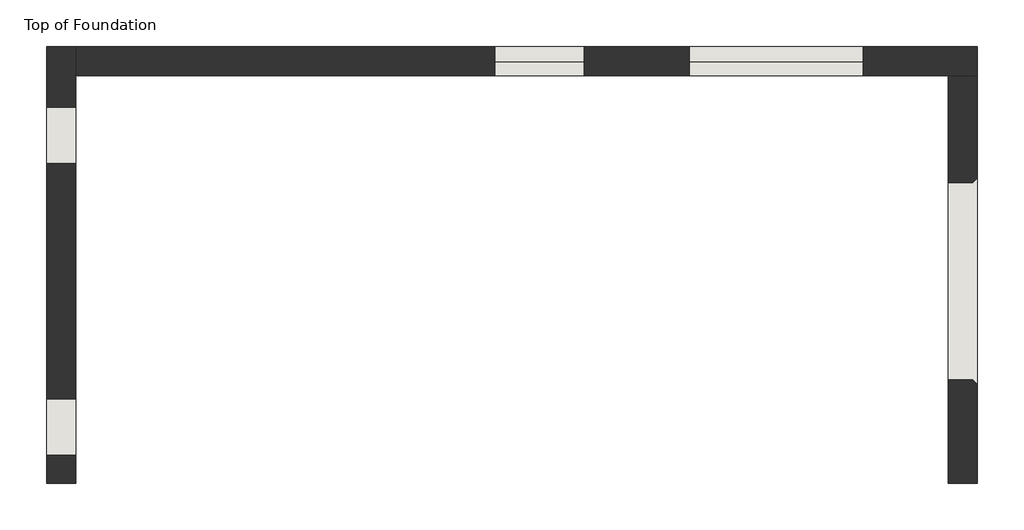
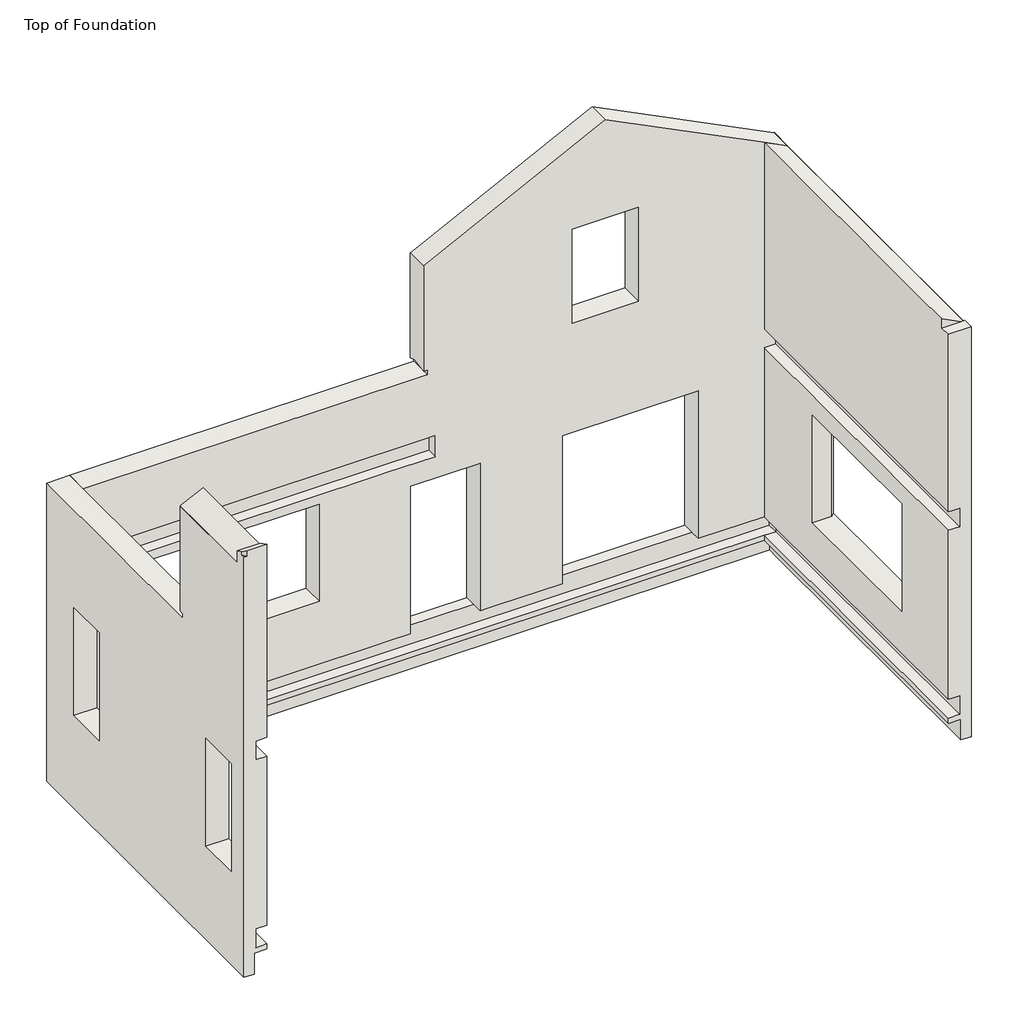
# One storey: 3 walls.
"""IFC4 building model written with IfcOpenShell, lengths in millimetres."""

from ifc_helpers import new_model, si_unit, origin, place, context, project, spatial, faceted_brep, element, save

model = new_model("IFC4")

# Units and contexts
model_context = context("Model", 3, world=origin())
ifc_project = project(units=[si_unit("LENGTHUNIT", "METRE", prefix="MILLI")], contexts=[model_context])

# Site, building, storey
site = spatial("IfcSite", under=ifc_project)
building = spatial("IfcBuilding", under=site)
storey = spatial("IfcBuildingStorey", under=building, Name="Top of Foundation", Elevation=-349.25)

# Walls
placement = place(None, origin())
element("IfcWall", 1, ObjectType="Exterior - Brick on Mtl. Stud", at=placement, inside=storey, context=model_context, shape_type="Brep", body=[
    faceted_brep([(-5671.6803068, 3152.0888758, -349.25), (-5671.6803068, 7558.9888758, -349.25), (-5671.6803068, 7876.4888758, -349.25), (-5671.6803068, 7876.4888758, 3708.4), (-5671.6803068, 7558.9888758, 3708.4), (-5671.6803068, 4676.0888758, 3708.4), (-5671.6803068, 4612.5888758, 3708.4), (-5671.6803068, 4612.5888758, 3774.0166667), (-5671.6803068, 4676.0888758, 3774.0166667), (-5671.6803068, 4676.0888758, 5468.9375), (-5671.6803068, 4358.5888758, 5468.9375), (-5671.6803068, 3304.4888758, 5468.9375), (-5671.6803068, 3304.4888758, 5488.5342644), (-5671.6803068, 3152.0888758, 5564.7342644), (-5671.6803068, 3152.0888758, 2743.2), (-5671.6803068, 4358.5888758, 2743.2), (-5671.6803068, 4514.1638758, 2743.2), (-5671.6803068, 4514.1638758, 2781.3), (-5671.6803068, 4676.0888758, 2781.3), (-5671.6803068, 7558.9888758, 2781.3), (-5671.6803068, 7714.5638758, 2781.3), (-5671.6803068, 7714.5638758, 2470.15), (-5671.6803068, 7558.9888758, 2470.15), (-5671.6803068, 3152.0888758, 2470.15), (-5671.6803068, 3152.0888758, 0.0), (-5671.6803068, 7558.9888758, 0.0), (-5671.6803068, 7714.5638758, 0.0), (-5671.6803068, 7714.5638758, -273.05), (-5671.6803068, 7558.9888758, -273.05), (-5671.6803068, 3152.0888758, -273.05), (-5671.6803068, 3456.8888758, 711.2), (-5671.6803068, 3456.8888758, 2286.0), (-5671.6803068, 4066.4888758, 2286.0), (-5671.6803068, 4066.4888758, 711.2), (-5671.6803068, 6609.6638758, 711.2), (-5671.6803068, 6609.6638758, 2286.0), (-5671.6803068, 7219.2638758, 2286.0), (-5671.6803068, 7219.2638758, 711.2), (-5989.1803068, 3152.0888758, -654.05), (-5989.1803068, 3152.0888758, 5486.4), (-5989.1803068, 3199.7138758, 5486.4), (-5989.1803068, 3199.7138758, 5540.9217644), (-5989.1803068, 3304.4888758, 5488.5342644), (-5989.1803068, 3304.4888758, 5312.3217644), (-5989.1803068, 4676.0888758, 5312.3217644), (-5989.1803068, 4676.0888758, 3779.52), (-5989.1803068, 4612.5888758, 3779.52), (-5989.1803068, 4612.5888758, 3708.4), (-5989.1803068, 7876.4888758, 3708.4), (-5989.1803068, 7876.4888758, -654.05), (-5989.1803068, 3456.8888758, 2286.0), (-5989.1803068, 3456.8888758, 711.2), (-5989.1803068, 4066.4888758, 711.2), (-5989.1803068, 4066.4888758, 2286.0), (-5989.1803068, 6609.6638758, 2286.0), (-5989.1803068, 6609.6638758, 711.2), (-5989.1803068, 7219.2638758, 711.2), (-5989.1803068, 7219.2638758, 2286.0), (-5846.3053068, 3152.0888758, -654.05), (-5846.3053068, 3152.0888758, -349.25), (-5684.3803068, 3152.0888758, -349.25), (-5827.2553068, 3152.0888758, -273.05), (-5827.2553068, 3152.0888758, 0.0), (-5827.2553068, 3152.0888758, 2470.15), (-5827.2553068, 3152.0888758, 2743.2), (-5941.5553068, 3152.0888758, 5564.7342644), (-5941.5553068, 3152.0888758, 5486.4), (-5984.911778, 4676.0888758, 5312.3217644), (-5887.5803068, 4676.0888758, 3810.0), (-5846.3053068, 7876.4888758, -349.25), (-5846.3053068, 7876.4888758, -654.05), (-5937.286778, 3304.4888758, 5336.1342644), (-5984.911778, 3304.4888758, 5312.3217644), (-5846.3053068, 7733.6138758, -349.25), (-5846.3053068, 7733.6138758, -654.05), (-5827.2553068, 7714.5638758, -273.05), (-5827.2553068, 7714.5638758, 0.0), (-5827.2553068, 7714.5638758, 2470.15), (-5827.2553068, 4514.1638758, 2470.15), (-5827.2553068, 4514.1638758, 2743.2), (-5827.2553068, 7714.5638758, 2781.3), (-5827.2553068, 4514.1638758, 2781.3), (-5887.5803068, 4612.5888758, 3810.0)], [[[0, 1, 2, 3, 4, 5, 6, 7, 8, 9, 10, 11, 12, 13, 14, 15, 16, 17, 18, 19, 20, 21, 22, 23, 24, 25, 26, 27, 28, 29], [30, 31, 32, 33], [34, 35, 36, 37]], [[38, 39, 40, 41, 42, 43, 44, 45, 46, 47, 48, 49], [50, 51, 52, 53], [54, 55, 56, 57]], [[39, 38, 58, 59, 60, 0, 29, 61, 62, 24, 23, 63, 64, 14, 13, 65, 66]], [[3, 48, 47, 6, 5, 4]], [[67, 9, 8, 68, 45, 44]], [[3, 2, 69, 70, 49, 48]], [[43, 42, 12, 11, 71, 72]], [[40, 39, 66]], [[40, 66, 65, 41]], [[11, 10, 9, 67, 72, 71]], [[44, 43, 72, 67]], [[13, 12, 42, 41, 65]], [[2, 1, 0, 60, 59, 73, 69]], [[69, 73, 59, 58, 74, 70]], [[58, 38, 49, 70, 74]], [[51, 50, 31, 30]], [[52, 51, 30, 33]], [[53, 52, 33, 32]], [[50, 53, 32, 31]], [[55, 54, 35, 34]], [[56, 55, 34, 37]], [[57, 56, 37, 36]], [[54, 57, 36, 35]], [[75, 61, 29, 28, 27]], [[76, 26, 25, 24, 62]], [[76, 75, 27, 26]], [[75, 76, 62, 61]], [[63, 23, 22, 21, 77, 78]], [[64, 79, 16, 15, 14]], [[79, 64, 63, 78, 77, 80, 81]], [[81, 80, 20, 19, 18, 17]], [[80, 77, 21, 20]], [[79, 81, 17, 16]], [[6, 47, 46, 82, 7]], [[7, 82, 68, 8]], [[82, 46, 45, 68]]]),
])
element("IfcWall", 2, ObjectType="Exterior - Brick on Mtl. Stud", at=placement, inside=storey, context=model_context, shape_type="Brep", body=[
    faceted_brep([(-5671.6803068, 7558.9888758, -349.25), (3751.7196932, 7558.9888758, -349.25), (4069.2196932, 7558.9888758, -349.25), (4069.2196932, 7558.9888758, 5312.3217644), (4064.9511643, 7558.9888758, 5312.3217644), (3751.7196932, 7558.9888758, 5468.9375), (1554.6196932, 7558.9888758, 6567.4875), (-642.4803068, 7558.9888758, 5468.9375), (-955.711778, 7558.9888758, 5312.3217644), (-959.9803068, 7558.9888758, 5312.3217644), (-959.9803068, 7558.9888758, 3774.0166667), (-909.1803068, 7558.9888758, 3774.0166667), (-909.1803068, 7558.9888758, 3708.4), (-959.9803068, 7558.9888758, 3708.4), (-5671.6803068, 7558.9888758, 3708.4), (-5671.6803068, 7558.9888758, 2781.3), (-959.9803068, 7558.9888758, 2781.3), (-798.0553068, 7558.9888758, 2781.3), (-798.0553068, 7558.9888758, 2743.2), (-798.0553068, 7558.9888758, 2470.15), (-1480.6803068, 7558.9888758, 2470.15), (-1601.3303068, 7558.9888758, 2470.15), (-5671.6803068, 7558.9888758, 2470.15), (-5671.6803068, 7558.9888758, 0.0), (-1601.3303068, 7558.9888758, 0.0), (-1480.6803068, 7558.9888758, 0.0), (-1144.1303068, 7558.9888758, 0.0), (-1144.1303068, 7558.9888758, 2159.0), (-178.9303068, 7558.9888758, 2159.0), (-178.9303068, 7558.9888758, 0.0), (-77.3303068, 7558.9888758, 0.0), (43.3196932, 7558.9888758, 0.0), (957.7196932, 7558.9888758, 0.0), (957.7196932, 7558.9888758, 2159.0), (2837.3196932, 7558.9888758, 2159.0), (2837.3196932, 7558.9888758, 0.0), (3751.7196932, 7558.9888758, 0.0), (3907.2946932, 7558.9888758, 0.0), (3907.2946932, 7558.9888758, -273.05), (3751.7196932, 7558.9888758, -273.05), (-5671.6803068, 7558.9888758, -273.05), (1097.4196932, 7558.9888758, 3759.2), (1097.4196932, 7558.9888758, 5130.8), (2011.8196932, 7558.9888758, 5130.8), (2011.8196932, 7558.9888758, 3759.2), (-2399.8428068, 7558.9888758, 2336.8), (-2399.8428068, 7558.9888758, 914.4), (-4838.2428068, 7558.9888758, 914.4), (-4838.2428068, 7558.9888758, 2336.8), (4069.2196932, 7876.4888758, 5312.3217644), (4069.2196932, 7876.4888758, -654.05), (-4312.7803068, 7876.4888758, -654.05), (-5684.3803068, 7876.4888758, -654.05), (-5846.3053068, 7876.4888758, -654.05), (-5846.3053068, 7876.4888758, -349.25), (-5671.6803068, 7876.4888758, -349.25), (-5671.6803068, 7876.4888758, 3708.4), (-909.1803068, 7876.4888758, 3708.4), (-909.1803068, 7876.4888758, 3779.52), (-959.9803068, 7876.4888758, 3779.52), (-959.9803068, 7876.4888758, 5312.3217644), (-955.711778, 7876.4888758, 5312.3217644), (1554.6196932, 7876.4888758, 6567.4875), (4064.9511643, 7876.4888758, 5312.3217644), (1097.4196932, 7876.4888758, 5130.8), (1097.4196932, 7876.4888758, 3759.2), (2011.8196932, 7876.4888758, 3759.2), (2011.8196932, 7876.4888758, 5130.8), (-1144.1303068, 7876.4888758, 2159.0), (-1144.1303068, 7876.4888758, 0.0), (-178.9303068, 7876.4888758, 0.0), (-178.9303068, 7876.4888758, 2159.0), (-2399.8428068, 7876.4888758, 914.4), (-2399.8428068, 7876.4888758, 2336.8), (-4838.2428068, 7876.4888758, 2336.8), (-4838.2428068, 7876.4888758, 914.4), (2837.3196932, 7876.4888758, 0.0), (2837.3196932, 7876.4888758, 2159.0), (957.7196932, 7876.4888758, 2159.0), (957.7196932, 7876.4888758, 0.0), (4069.2196932, 7571.6888758, -349.25), (4069.2196932, 7733.6138758, -349.25), (4069.2196932, 7733.6138758, -654.05), (-959.9803068, 7774.8888758, 3810.0), (-5671.6803068, 7733.6138758, -349.25), (-5671.6803068, 7714.5638758, -273.05), (-5671.6803068, 7714.5638758, 0.0), (-5671.6803068, 7714.5638758, 2470.15), (-5671.6803068, 7714.5638758, 2781.3), (-4312.7803068, 7733.6138758, -349.25), (3926.3446932, 7733.6138758, -349.25), (-5684.3803068, 7733.6138758, -349.25), (-5846.3053068, 7733.6138758, -349.25), (-5846.3053068, 7733.6138758, -654.05), (-5684.3803068, 7733.6138758, -654.05), (-4312.7803068, 7733.6138758, -654.05), (3926.3446932, 7733.6138758, -654.05), (-1144.1303068, 7714.5638758, 0.0), (-178.9303068, 7714.5638758, 0.0), (2837.3196932, 7714.5638758, 0.0), (957.7196932, 7714.5638758, 0.0), (-798.0553068, 7714.5638758, 2470.15), (-798.0553068, 7714.5638758, 2781.3), (3907.2946932, 7714.5638758, -273.05), (3907.2946932, 7714.5638758, 0.0), (-909.1803068, 7774.8888758, 3810.0)], [[[0, 1, 2, 3, 4, 5, 6, 7, 8, 9, 10, 11, 12, 13, 14, 15, 16, 17, 18, 19, 20, 21, 22, 23, 24, 25, 26, 27, 28, 29, 30, 31, 32, 33, 34, 35, 36, 37, 38, 39, 40], [41, 42, 43, 44], [45, 46, 47, 48]], [[49, 50, 51, 52, 53, 54, 55, 56, 57, 58, 59, 60, 61, 62, 63], [64, 65, 66, 67], [68, 69, 70, 71], [72, 73, 74, 75], [76, 77, 78, 79]], [[3, 2, 80, 81, 82, 50, 49]], [[12, 57, 56, 14, 13]], [[9, 60, 59, 83, 10]], [[14, 56, 55, 84, 0, 40, 85, 86, 23, 22, 87, 88, 15]], [[60, 9, 8, 61]], [[8, 7, 6, 62, 61]], [[6, 5, 4, 63, 62]], [[3, 49, 63, 4]], [[2, 1, 0, 84, 89, 90, 81, 80]], [[81, 90, 89, 84, 91, 92, 93, 94, 95, 96, 82]], [[50, 82, 96, 95, 94, 93, 53, 52, 51]], [[92, 91, 84, 55, 54]], [[53, 93, 92, 54]], [[65, 64, 42, 41]], [[66, 65, 41, 44]], [[67, 66, 44, 43]], [[64, 67, 43, 42]], [[68, 27, 26, 97, 69]], [[27, 68, 71, 28]], [[28, 71, 70, 98, 29]], [[70, 69, 97, 98]], [[46, 72, 75, 47]], [[73, 45, 48, 74]], [[72, 46, 45, 73]], [[74, 48, 47, 75]], [[34, 77, 76, 99, 35]], [[77, 34, 33, 78]], [[78, 33, 32, 100, 79]], [[76, 79, 100, 99]], [[19, 101, 87, 22, 21, 20]], [[88, 102, 17, 16, 15]], [[101, 102, 88, 87]], [[102, 101, 19, 18, 17]], [[38, 103, 85, 40, 39]], [[99, 104, 37, 36, 35]], [[98, 100, 32, 31, 30, 29]], [[86, 97, 26, 25, 24, 23]], [[103, 104, 99, 100, 98, 97, 86, 85]], [[104, 103, 38, 37]], [[11, 105, 58, 57, 12]], [[105, 11, 10, 83]], [[58, 105, 83, 59]]]),
])
element("IfcWall", 3, ObjectType="Exterior - Brick on Mtl. Stud", at=placement, inside=storey, context=model_context, shape_type="Brep", body=[
    faceted_brep([(3751.7196932, 7558.9888758, -349.25), (3751.7196932, 3152.0888758, -349.25), (3751.7196932, 3152.0888758, -273.05), (3751.7196932, 7558.9888758, -273.05), (3751.7196932, 3304.4888758, 5336.1342644), (3751.7196932, 3304.4888758, 5468.9375), (3751.7196932, 3844.2388758, 5468.9375), (3751.7196932, 3964.8888758, 5468.9375), (3751.7196932, 7558.9888758, 5468.9375), (3751.7196932, 7558.9888758, 2743.2), (3751.7196932, 3964.8888758, 2743.2), (3751.7196932, 3844.2388758, 2743.2), (3751.7196932, 3152.0888758, 2743.2), (3751.7196932, 3152.0888758, 5336.1342644), (3751.7196932, 7558.9888758, 0.0), (3751.7196932, 3152.0888758, 0.0), (3751.7196932, 3152.0888758, 2470.15), (3751.7196932, 7558.9888758, 2470.15), (3751.7196932, 6404.8763758, 2184.4), (3751.7196932, 4271.2763758, 2184.4), (3751.7196932, 4271.2763758, 609.6), (3751.7196932, 6404.8763758, 609.6), (4069.2196932, 3152.0888758, 5336.1342644), (4069.2196932, 3152.0888758, -654.05), (4069.2196932, 7571.6888758, -654.05), (4069.2196932, 7733.6138758, -654.05), (4069.2196932, 7733.6138758, -349.25), (4069.2196932, 7558.9888758, -349.25), (4069.2196932, 7558.9888758, 5312.3217644), (4069.2196932, 3304.4888758, 5312.3217644), (4069.2196932, 3304.4888758, 5336.1342644), (4069.2196932, 4221.8849671, 2184.4), (4069.2196932, 6454.2677845, 2184.4), (4069.2196932, 6454.2677845, 609.6), (4069.2196932, 4221.8849671, 609.6), (3907.2946932, 3152.0888758, 2743.2), (3907.2946932, 3152.0888758, 2470.15), (3907.2946932, 3152.0888758, 0.0), (3907.2946932, 3152.0888758, -273.05), (3764.4196932, 3152.0888758, -349.25), (3926.3446932, 3152.0888758, -349.25), (3926.3446932, 3152.0888758, -654.05), (4064.9511643, 7558.9888758, 5312.3217644), (3926.3446932, 7558.9888758, -349.25), (3907.2946932, 7558.9888758, -273.05), (3907.2946932, 7558.9888758, 0.0), (3907.2946932, 7558.9888758, 2470.15), (3907.2946932, 7558.9888758, 2743.2), (4064.9511643, 3304.4888758, 5312.3217644), (4017.3261643, 3304.4888758, 5336.1342644), (3926.3446932, 7571.6888758, -349.25), (3926.3446932, 7733.6138758, -349.25), (3926.3446932, 7733.6138758, -654.05), (3926.3446932, 7571.6888758, -654.05), (4019.8282845, 6404.8763758, 2184.4), (4019.8282845, 4271.2763758, 2184.4), (4019.8282845, 6404.8763758, 609.6), (4019.8282845, 4271.2763758, 609.6)], [[[0, 1, 2, 3]], [[4, 5, 6, 7, 8, 9, 10, 11, 12, 13]], [[14, 15, 16, 17], [18, 19, 20, 21]], [[22, 23, 24, 25, 26, 27, 28, 29, 30], [31, 32, 33, 34]], [[23, 22, 13, 12, 35, 36, 16, 15, 37, 38, 2, 1, 39, 40, 41]], [[42, 28, 27, 43, 0, 3, 44, 45, 14, 17, 46, 47, 9, 8]], [[30, 29, 48, 49]], [[4, 13, 22, 30, 49]], [[8, 7, 6, 5, 49, 48, 42]], [[29, 28, 42, 48]], [[5, 4, 49]], [[1, 0, 43, 40, 39]], [[40, 43, 50, 51, 52, 53, 41]], [[23, 41, 53, 52, 25, 24]], [[51, 50, 43, 27, 26]], [[25, 52, 51, 26]], [[54, 32, 31, 55, 19, 18]], [[56, 21, 20, 57, 34, 33]], [[54, 18, 21, 56]], [[19, 55, 57, 20]], [[55, 31, 34, 57]], [[32, 54, 56, 33]], [[38, 44, 3, 2]], [[45, 37, 15, 14]], [[44, 38, 37, 45]], [[36, 46, 17, 16]], [[47, 35, 12, 11, 10, 9]], [[46, 36, 35, 47]]]),
])

save(model, "model.ifc")

# Revit data of these elements
# Type "Exterior - Brick on Mtl. Stud"
#   Assembly Code = "B2010158"
#   Layers, outside or top first: 0' - 3 5/8" "Brick, Common" (function 4); 0' - 2" "Air" (function 3); 0' - 0" "Air Infiltration Barrier" (function 100); 0' - 0 3/4" "Plywood, Sheathing" (function 2); 0' - 5 1/2" "Metal Stud Layer" (function 1); 0' - 0" "Vapor Retarder" (function 100); 0' - 0 5/8" "Gypsum Wall Board" (function 5)
# Elements 1, 2 (IfcWall, "Exterior - Brick on Mtl. Stud")
#   built-in parameter 1012829 = -1 (stored number, unit not read)
#   Top Offset = 0' - 0"
#   Base Offset = 0' - 0"
#   wall height = 19' - 1 3/4"
#   Phase Created = New Construction
#   Base Constraint = Top of Foundation
#   Top Constraint = Roof
#   Materials on its faces: "Default Wall", "Brick, Common", "Gypsum Wall Board"
# Element 3 (IfcWall, "Exterior - Brick on Mtl. Stud")
#   built-in parameter 1012829 = -1 (stored number, unit not read)
#   Top Offset = 0' - 0"
#   Base Offset = 0' - 0"
#   wall height = 19' - 1 3/4"
#   Phase Created = New Construction
#   Base Constraint = Top of Foundation
#   Top Constraint = Roof
#   Materials on its faces: "Default Wall", "Gypsum Wall Board", "Brick, Common"
# Materials
#   "Brick, Common": class "Masonry", colour RGB 140 101 80, transparency 0, Keynote = "04 21 00.A1", Description = "Common brick", Cost = 0
#   "Air": class "Gas", colour RGB 255 255 255, transparency 0, Description = "Air", Cost = 0
#   "Air Infiltration Barrier": class "Generic", colour RGB 127 127 127, transparency 0, Description = "physical material", Cost = 0
#   "Plywood, Sheathing": class "Wood", colour RGB 193 140 64, transparency 0, Description = "Plywood, sheathing grade", Cost = 0
#   "Metal Stud Layer": class "Metal", colour RGB 199 199 199, transparency 0, Description = "Light gauge steel framing, thermal air layer", Cost = 0
#   "Vapor Retarder": class "Generic", colour RGB 127 127 127, transparency 0, Description = "Polyethylene film membrane", Cost = 0
#   "Gypsum Wall Board": class "Generic", colour RGB 127 127 127, transparency 0, Description = "Gypsum Wall Board", Cost = 0
#   "Default Wall": class "Miscellaneous", colour RGB 128 128 128, transparency 0, Cost = 0
